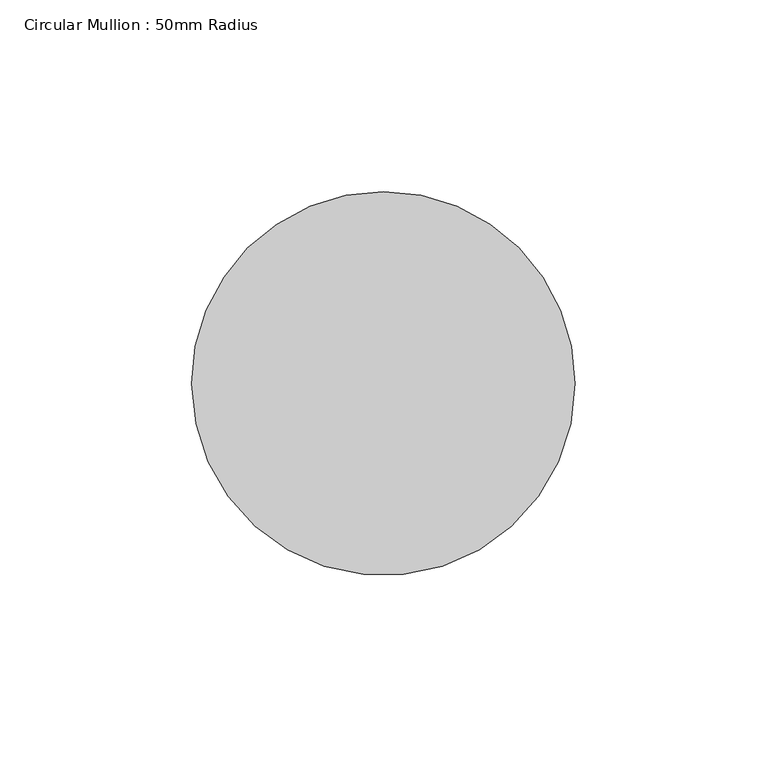
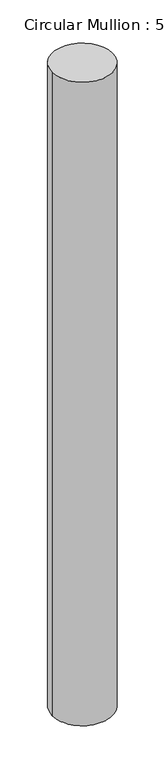
"""IFC4 building model written with IfcOpenShell, lengths in millimetres: member geometry, Circular Mullion : 50mm Radius."""

import ifcopenshell
import ifcopenshell.guid

model = None  # the IFC model being written
_history = None  # IfcOwnerHistory: only IFC2X3 demands one
_inside = {}  # id of a spatial element -> (the spatial element, [elements in it])
_under = {}  # id of a project, library or spatial element -> (it, [spatial elements below it])
_declared = {}  # id of a project -> (the project, [libraries it declares])
_typed = {}  # id of a type object -> (the type object, [elements of that type])
_made_of = {}  # id of a material, layer set ... -> (it, [elements and type objects made of it])


def new_model(schema):
    """Start an empty IFC model of exactly this schema.

    Asked for "IFC4X3", IfcOpenShell would pick the latest addendum, in which some entities
    have other attributes; the version numbers below select the first issue.
    IFC2X3 requires an IfcOwnerHistory on every rooted entity: one is made here for all.
    """
    global model, _history
    if schema == "IFC4X3":
        model = ifcopenshell.file(schema_version=(4, 3, 0, 0))
    else:
        model = ifcopenshell.file(schema=schema)
    _inside.clear()
    _under.clear()
    _declared.clear()
    _typed.clear()
    _made_of.clear()
    _history = None
    if model.schema == "IFC2X3":
        org = make("IfcOrganization", Name="unknown")
        user = make(
            "IfcPersonAndOrganization",
            ThePerson=make("IfcPerson", FamilyName="unknown"),
            TheOrganization=org,
        )
        app = make(
            "IfcApplication",
            ApplicationDeveloper=org,
            Version="unknown",
            ApplicationFullName="unknown",
            ApplicationIdentifier="unknown",
        )
        _history = make(
            "IfcOwnerHistory",
            OwningUser=user,
            OwningApplication=app,
            ChangeAction="ADDED",
            CreationDate=0,
        )
    return model


def make(cls, **values):
    """One entity of the class cls with the attributes given. An attribute that is None is left unset."""
    return model.create_entity(
        cls, **{name: value for name, value in values.items() if value is not None}
    )


def rooted(cls, **values):
    """An entity with a GlobalId (a new one), such as an element, a storey or a relation."""
    return make(cls, GlobalId=ifcopenshell.guid.new(), OwnerHistory=_history, **values)


def si_unit(unit_type, name, prefix=None):
    """IfcSIUnit, for example si_unit("LENGTHUNIT", "METRE", prefix="MILLI")."""
    return make("IfcSIUnit", UnitType=unit_type, Prefix=prefix, Name=name)


def assignment(units):
    """IfcUnitAssignment: the units of a project."""
    return None if units is None else make("IfcUnitAssignment", Units=units)


def point(xyz):
    """IfcCartesianPoint."""
    return None if xyz is None else make("IfcCartesianPoint", Coordinates=xyz)


def direction(xyz):
    """IfcDirection."""
    return None if xyz is None else make("IfcDirection", DirectionRatios=xyz)


def frame(location, z_axis=None, x_axis=None):
    """IfcAxis2Placement3D, a coordinate frame: its origin and axes. An axis left out is left unset."""
    return make(
        "IfcAxis2Placement3D",
        Location=point(location),
        Axis=direction(z_axis),
        RefDirection=direction(x_axis),
    )


def origin():
    """The frame at (0, 0, 0) with its axes left unset."""
    return frame((0.0, 0.0, 0.0))


def place(relative_to, where):
    """IfcLocalPlacement: puts the frame where relative to a parent placement (None: the world)."""
    return make(
        "IfcLocalPlacement", PlacementRelTo=relative_to, RelativePlacement=where
    )


def context(
    kind, dimensions, precision=None, world=None, true_north=None, identifier=None
):
    """IfcGeometricRepresentationContext, for example the 3D "Model" context."""
    return make(
        "IfcGeometricRepresentationContext",
        ContextIdentifier=identifier,
        ContextType=kind,
        CoordinateSpaceDimension=dimensions,
        Precision=precision,
        WorldCoordinateSystem=world,
        TrueNorth=true_north,
    )


def project(units=None, contexts=None):
    """IfcProject with its units and contexts."""
    return rooted(
        "IfcProject",
        Name="project",
        RepresentationContexts=contexts,
        UnitsInContext=assignment(units),
    )


def spatial(cls, under=None, at=None, **own):
    """A site, building, storey or space (cls), placed at a placement, below another one or the project."""
    s = rooted(cls, ObjectPlacement=at, **own)
    if under is not None:
        _under.setdefault(under.id(), (under, []))[1].append(s)
    return s


def ellipse_curve(where, semi_axis1, semi_axis2):
    """IfcEllipse in the frame where."""
    return make(
        "IfcEllipse", Position=where, SemiAxis1=semi_axis1, SemiAxis2=semi_axis2
    )


def shape(context_of_items, identifier, shape_type, items):
    """IfcShapeRepresentation: the items that make up one representation, for example the "Body"."""
    return make(
        "IfcShapeRepresentation",
        ContextOfItems=context_of_items,
        RepresentationIdentifier=identifier,
        RepresentationType=shape_type,
        Items=items,
    )


def source(mapping_origin, context_of_items, identifier, shape_type, items):
    """IfcRepresentationMap: a shape defined once, which mapped items show again and again."""
    return make(
        "IfcRepresentationMap",
        MappingOrigin=mapping_origin,
        MappedRepresentation=shape(context_of_items, identifier, shape_type, items),
    )


def transform(
    local_origin,
    x_axis=None,
    y_axis=None,
    z_axis=None,
    scale=None,
    scale2=None,
    scale3=None,
    uniform=True,
):
    """IfcCartesianTransformationOperator3D, or its non-uniform kind. x_axis, y_axis, z_axis: its Axis1, 2, 3."""
    if uniform:
        return make(
            "IfcCartesianTransformationOperator3D",
            Axis1=direction(x_axis),
            Axis2=direction(y_axis),
            LocalOrigin=point(local_origin),
            Scale=scale,
            Axis3=direction(z_axis),
        )
    return make(
        "IfcCartesianTransformationOperator3DnonUniform",
        Axis1=direction(x_axis),
        Axis2=direction(y_axis),
        LocalOrigin=point(local_origin),
        Scale=scale,
        Axis3=direction(z_axis),
        Scale2=scale2,
        Scale3=scale3,
    )


def mapped(mapping_source, mapping_target):
    """IfcMappedItem: shows the shape of a source again, moved by a transform."""
    return make(
        "IfcMappedItem", MappingSource=mapping_source, MappingTarget=mapping_target
    )


def made_of(thing, what):
    """Note that an element or type object is made of a material, layer set ...; save() writes the relation."""
    if what is not None:
        _made_of.setdefault(what.id(), (what, []))[1].append(thing)
    return thing


def element(
    cls,
    number,
    at=None,
    inside=None,
    cuts=None,
    type_object=None,
    material=None,
    context=None,
    identifier="Body",
    shape_type=None,
    held_by="IfcProductDefinitionShape",
    body=None,
    shapes=None,
    **own,
):
    """One element of the class cls, such as IfcWall. Its Tag is "e" and its number.

    at: its placement. inside: the storey or other place that contains it. cuts: it is an
    opening in that element (IfcRelVoidsElement). A single representation is given by context,
    identifier, shape_type and body (its items); several are given by shapes. held_by: the class
    of the entity that holds the representations. save() writes the other relations.
    """
    e = rooted(cls, Tag="e%d" % number, ObjectPlacement=at, **own)
    if body is not None:
        shapes = [shape(context, identifier, shape_type, body)]
    if shapes is not None:
        e.Representation = make(held_by, Representations=shapes)
    if inside is not None:
        _inside.setdefault(inside.id(), (inside, []))[1].append(e)
    if cuts is not None:
        rooted(
            "IfcRelVoidsElement", RelatingBuildingElement=cuts, RelatedOpeningElement=e
        )
    if type_object is not None:
        _typed.setdefault(type_object.id(), (type_object, []))[1].append(e)
    return made_of(e, material)


def aggregate(whole, parts):
    """IfcRelAggregates: a whole, such as a stair, and the parts it consists of."""
    return rooted("IfcRelAggregates", RelatingObject=whole, RelatedObjects=parts)


def save(model, path):
    """Write the relations noted so far, then the file.

    IfcRelAggregates (storeys below a building ...), IfcRelContainedInSpatialStructure (elements
    in a storey), IfcRelDefinesByType, IfcRelAssociatesMaterial and IfcRelDeclares: one each for
    every whole, place, type object, material and project.
    """
    for whole, parts in _under.values():
        aggregate(whole, parts)
    for where, things in _inside.values():
        rooted(
            "IfcRelContainedInSpatialStructure",
            RelatedElements=things,
            RelatingStructure=where,
        )
    for kind, things in _typed.values():
        rooted("IfcRelDefinesByType", RelatedObjects=things, RelatingType=kind)
    for what, things in _made_of.values():
        rooted("IfcRelAssociatesMaterial", RelatedObjects=things, RelatingMaterial=what)
    for by, libraries in _declared.values():
        rooted("IfcRelDeclares", RelatingContext=by, RelatedDefinitions=libraries)
    model.write(path)


def plane_surface(at):
    """IfcPlane: the flat surface through the origin of the frame at, square to its z axis."""
    return make("IfcPlane", Position=at)


def cylinder_surface(at, radius):
    """IfcCylindricalSurface: all points at the distance radius from the z axis of the frame at."""
    return make("IfcCylindricalSurface", Position=at, Radius=radius)


def advanced_brep(points, edges, surfaces, faces):
    """IfcAdvancedBrep: a solid bounded by faces that lie on surfaces and meet in shared edges.

    An edge is (start, end): straight between two places in points (the first is 0);
    or (start, end, curve); or (start, end, curve, False) where it runs against its curve.
    A face is (place in surfaces, loops), or (place, loops, False) where it looks against
    its surface's normal. A loop lists edges by number (the first is 1), with a minus sign
    where the edge is run from its end to its start. The first loop is the outer one.
    """
    corners = [point(p) for p in points]
    vertices = [make("IfcVertexPoint", VertexGeometry=c) for c in corners]
    made = []
    for start, end, *more in edges:
        made.append(
            make(
                "IfcEdgeCurve",
                EdgeStart=vertices[start],
                EdgeEnd=vertices[end],
                EdgeGeometry=more[0] if more else make("IfcPolyline", Points=[corners[start], corners[end]]),
                SameSense=more[1] if len(more) > 1 else True,
            )
        )
    hull = []
    for where, loops, *sense in faces:
        bounds = []
        for j, loop in enumerate(loops):
            ring = [make("IfcOrientedEdge", EdgeElement=made[abs(k) - 1], Orientation=k > 0) for k in loop]
            bounds.append(
                make(
                    "IfcFaceOuterBound" if j == 0 else "IfcFaceBound",
                    Bound=make("IfcEdgeLoop", EdgeList=ring),
                    Orientation=True,
                )
            )
        hull.append(make("IfcAdvancedFace", Bounds=bounds, FaceSurface=surfaces[where], SameSense=sense[0] if sense else True))
    return make("IfcAdvancedBrep", Outer=make("IfcClosedShell", CfsFaces=hull))


def circular_mullion_50mm_radius_870a85af(model_context):
    return source(origin(), model_context, "Body", "AdvancedBrep", [
        advanced_brep(
        [(-100.0, 0.0, 1.0191577), (0.0, 0.0, 0.0), (0.0, 0.0, -1123.3955871), (-100.0, 0.0, -1124.4515328)],
        [
            (0, 1, ellipse_curve(frame((-50.0, 0.0, 0.5095788), z_axis=(-0.010189950388839549, -0.01467413210080617, -0.9998404046437417), x_axis=(-0.5702889518304459, -0.8212498682972755, 0.01786519638399624)), 50.007981, 50.0)),
            (1, 2),
            (2, 3, ellipse_curve(frame((-50.0, 0.0, -1123.9235599), z_axis=(-0.010557647802399124, -0.015203638154693083, 0.9998286780542665), x_axis=(0.5702822632185547, 0.8212402362999913, 0.01850984981726201)), 50.0085676, 50.0)),
            (3, 0),
            (1, 0, ellipse_curve(frame((-50.0, 0.0, 0.5095788), z_axis=(-0.010189950388839549, -0.01467413210080617, -0.9998404046437417), x_axis=(-0.5702889518304459, -0.8212498682972755, 0.01786519638399624)), 50.007981, 50.0)),
            (3, 2, ellipse_curve(frame((-50.0, 0.0, -1123.9235599), z_axis=(-0.010557647802399124, -0.015203638154693083, 0.9998286780542665), x_axis=(0.5702822632185547, 0.8212402362999913, 0.01850984981726201)), 50.0085676, 50.0)),
        ],
        [
            cylinder_surface(frame((-50.0, 0.0, 0.0), z_axis=(0.0, 0.0, 1.0), x_axis=(1.0, 0.0, 0.0)), 50.0),
            plane_surface(frame((-250.3569157, 173.8518185, 0.0), z_axis=(0.010189950388839549, 0.01467413210080617, 0.9998404046437417), x_axis=(0.5702889518304458, 0.8212498682972756, -0.017865196384000973))),
            plane_surface(frame((-250.3569157, 173.8518185, -1123.3955871), z_axis=(0.010557647802399123, 0.01520363815469308, -0.9998286780542662), x_axis=(0.5702822632185546, 0.8212402362999909, 0.01850984981728221))),
        ],
        [
            (0, [[1, 2, 3, 4]]),
            (0, [[5, -4, 6, -2]]),
            (1, [[-1, -5]]),
            (2, [[-6, -3]]),
        ],
    ),
    ])


if __name__ == "__main__":
    model = new_model("IFC4")
    model_context = context("Model", 3, world=origin())
    ifc_project = project(units=[si_unit("LENGTHUNIT", "METRE", prefix="MILLI")], contexts=[model_context])
    site = spatial("IfcSite", under=ifc_project)
    building = spatial("IfcBuilding", under=site)
    placement = place(None, origin())
    circular_mullion_50mm_radius_shape = circular_mullion_50mm_radius_870a85af(model_context)
    element("IfcMember", 1, ObjectType="Circular Mullion : 50mm Radius", at=placement, inside=building, context=model_context, shape_type="MappedRepresentation", body=[
        mapped(circular_mullion_50mm_radius_shape, transform((0.0, 0.0, 0.0), x_axis=(1.0, 0.0, 0.0), y_axis=(0.0, 1.0, 0.0), z_axis=(0.0, 0.0, 1.0))),
    ])
    save(model, "model.ifc")

# Revit data of these elements
# Type "Circular Mullion : 50mm Radius"
#   built-in parameter 1007350 = 0.164042 (stored number, unit not read)
# Element 1 (IfcMember, "Circular Mullion : 50mm Radius")
#   Materials on its faces: "Aluminium"
# Materials
#   "Aluminium": class "Metal", colour RGB 247 247 247, transparency 0, Description = "Aluminium 6061", Cost = 0
